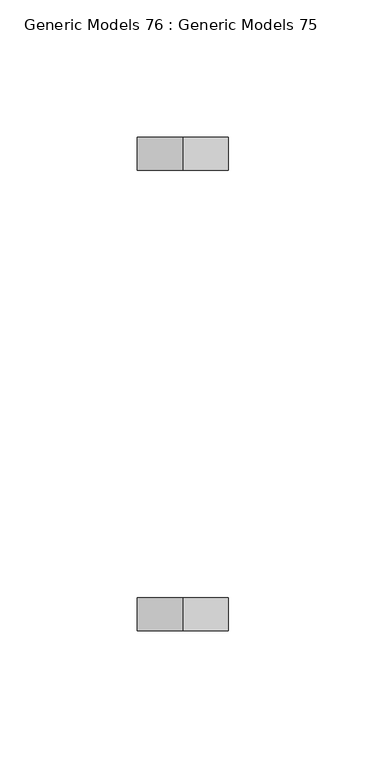
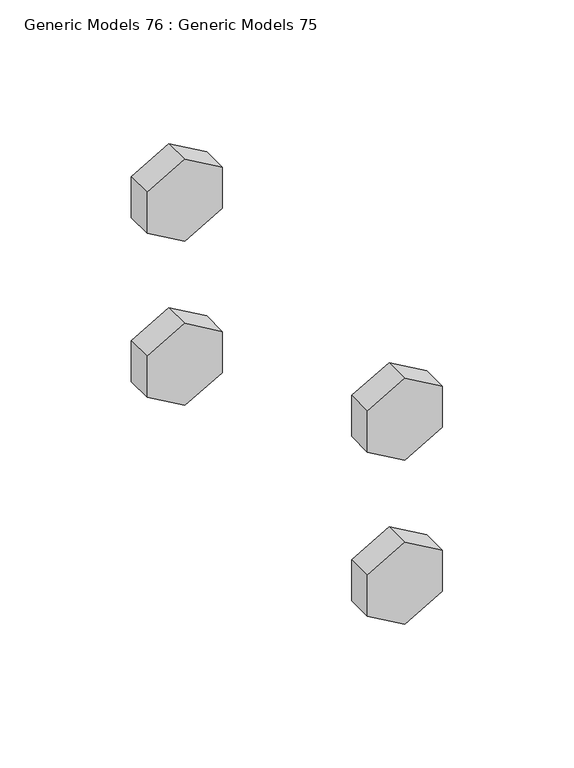
"""IFC4 building model written with IfcOpenShell, lengths in millimetres: proxy geometry, Generic Models 76 : Generic Models 75."""

from ifc_helpers import new_model, si_unit, frame, origin, place, context, project, spatial, polyline, outline, extrude, source, transform, mapped, element, save


def generic_models_76_generic_models_75_43fec320(model_context):
    return source(origin(), model_context, "Body", "SweptSolid", [
        extrude(outline(polyline([(271626.0125, 31991.9073871), (271645.0625, 31991.9073871), (271654.5875, 31975.4096032), (271645.0625, 31958.9118192), (271626.0125, 31958.9118192), (271616.4875, 31975.4096032), (271626.0125, 31991.9073871)])), frame((0.0, 30852.1281612, 0.0), z_axis=(0.0, 1.0, 0.0), x_axis=(0.0, 0.0, 1.0)), (0.0, 0.0, 1.0), 11.90625),
        extrude(outline(polyline([(271549.8125, 31991.9073871), (271568.8625, 31991.9073871), (271578.3875, 31975.4096032), (271568.8625, 31958.9118192), (271549.8125, 31958.9118192), (271540.2875, 31975.4096032), (271549.8125, 31991.9073871)])), frame((0.0, 30852.1281612, 0.0), z_axis=(0.0, 1.0, 0.0), x_axis=(0.0, 0.0, 1.0)), (0.0, 0.0, 1.0), 11.90625),
        extrude(outline(polyline([(271626.0125, 31991.9073871), (271645.0625, 31991.9073871), (271654.5875, 31975.4096032), (271645.0625, 31958.9118192), (271626.0125, 31958.9118192), (271616.4875, 31975.4096032), (271626.0125, 31991.9073871)])), frame((0.0, 30684.6469112, 0.0), z_axis=(0.0, 1.0, 0.0), x_axis=(0.0, 0.0, 1.0)), (0.0, 0.0, 1.0), 11.90625),
        extrude(outline(polyline([(271549.8125, 31991.9073871), (271568.8625, 31991.9073871), (271578.3875, 31975.4096032), (271568.8625, 31958.9118192), (271549.8125, 31958.9118192), (271540.2875, 31975.4096032), (271549.8125, 31991.9073871)])), frame((0.0, 30684.6469112, 0.0), z_axis=(0.0, 1.0, 0.0), x_axis=(0.0, 0.0, 1.0)), (0.0, 0.0, 1.0), 11.90625),
    ])


if __name__ == "__main__":
    model = new_model("IFC4")
    model_context = context("Model", 3, world=origin())
    ifc_project = project(units=[si_unit("LENGTHUNIT", "METRE", prefix="MILLI")], contexts=[model_context])
    site = spatial("IfcSite", under=ifc_project)
    building = spatial("IfcBuilding", under=site)
    placement = place(None, origin())
    generic_models_76_generic_models_75_shape = generic_models_76_generic_models_75_43fec320(model_context)
    element("IfcBuildingElementProxy", 1, Name="Generic Models 76 : Generic Models 75", ObjectType="Generic Models 76 : Generic Models 75", at=placement, inside=building, context=model_context, shape_type="MappedRepresentation", body=[
        mapped(generic_models_76_generic_models_75_shape, transform((0.0, 0.0, 0.0), x_axis=(1.0, 0.0, 0.0), y_axis=(0.0, 1.0, 0.0), z_axis=(0.0, 0.0, 1.0))),
    ])
    save(model, "model.ifc")
